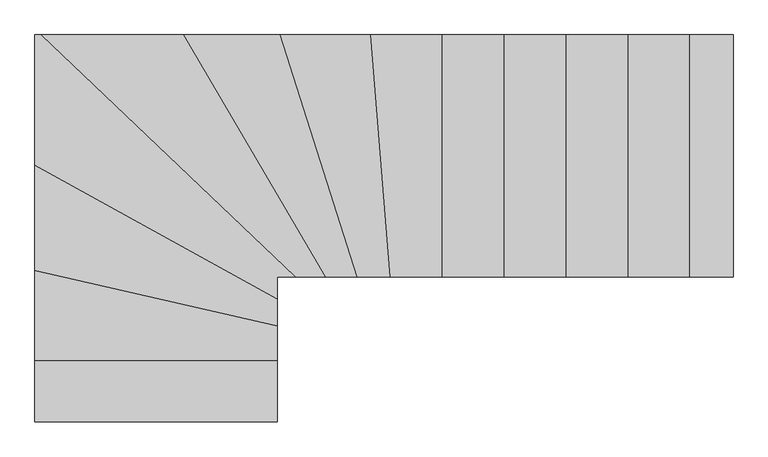
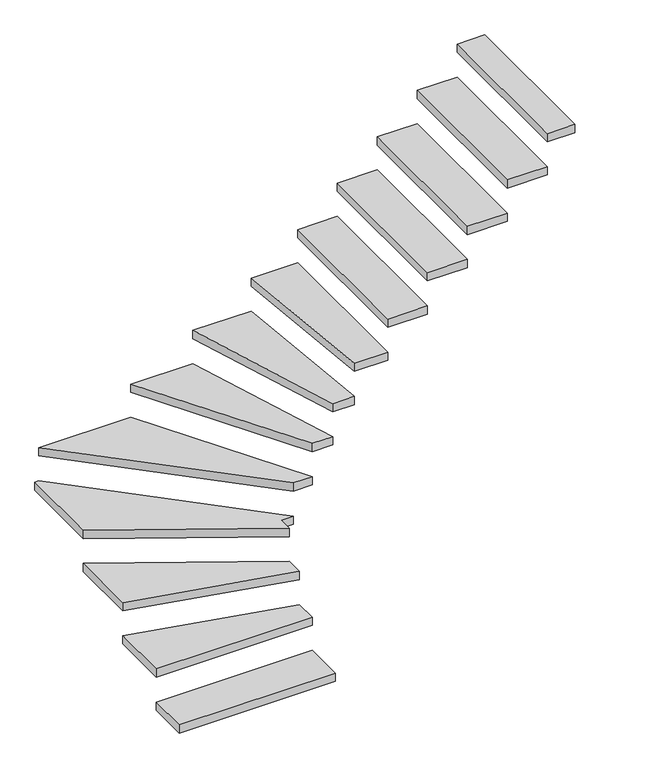
"""IFC4 building model written with IfcOpenShell, lengths in millimetres: stair geometry,   151260 :   151260."""

import ifcopenshell
import ifcopenshell.guid

model = None  # the IFC model being written
_history = None  # IfcOwnerHistory: only IFC2X3 demands one
_inside = {}  # id of a spatial element -> (the spatial element, [elements in it])
_under = {}  # id of a project, library or spatial element -> (it, [spatial elements below it])
_declared = {}  # id of a project -> (the project, [libraries it declares])
_typed = {}  # id of a type object -> (the type object, [elements of that type])
_made_of = {}  # id of a material, layer set ... -> (it, [elements and type objects made of it])


def new_model(schema):
    """Start an empty IFC model of exactly this schema.

    Asked for "IFC4X3", IfcOpenShell would pick the latest addendum, in which some entities
    have other attributes; the version numbers below select the first issue.
    IFC2X3 requires an IfcOwnerHistory on every rooted entity: one is made here for all.
    """
    global model, _history
    if schema == "IFC4X3":
        model = ifcopenshell.file(schema_version=(4, 3, 0, 0))
    else:
        model = ifcopenshell.file(schema=schema)
    _inside.clear()
    _under.clear()
    _declared.clear()
    _typed.clear()
    _made_of.clear()
    _history = None
    if model.schema == "IFC2X3":
        org = make("IfcOrganization", Name="unknown")
        user = make(
            "IfcPersonAndOrganization",
            ThePerson=make("IfcPerson", FamilyName="unknown"),
            TheOrganization=org,
        )
        app = make(
            "IfcApplication",
            ApplicationDeveloper=org,
            Version="unknown",
            ApplicationFullName="unknown",
            ApplicationIdentifier="unknown",
        )
        _history = make(
            "IfcOwnerHistory",
            OwningUser=user,
            OwningApplication=app,
            ChangeAction="ADDED",
            CreationDate=0,
        )
    return model


def make(cls, **values):
    """One entity of the class cls with the attributes given. An attribute that is None is left unset."""
    return model.create_entity(
        cls, **{name: value for name, value in values.items() if value is not None}
    )


def rooted(cls, **values):
    """An entity with a GlobalId (a new one), such as an element, a storey or a relation."""
    return make(cls, GlobalId=ifcopenshell.guid.new(), OwnerHistory=_history, **values)


def si_unit(unit_type, name, prefix=None):
    """IfcSIUnit, for example si_unit("LENGTHUNIT", "METRE", prefix="MILLI")."""
    return make("IfcSIUnit", UnitType=unit_type, Prefix=prefix, Name=name)


def assignment(units):
    """IfcUnitAssignment: the units of a project."""
    return None if units is None else make("IfcUnitAssignment", Units=units)


def point(xyz):
    """IfcCartesianPoint."""
    return None if xyz is None else make("IfcCartesianPoint", Coordinates=xyz)


def direction(xyz):
    """IfcDirection."""
    return None if xyz is None else make("IfcDirection", DirectionRatios=xyz)


def frame(location, z_axis=None, x_axis=None):
    """IfcAxis2Placement3D, a coordinate frame: its origin and axes. An axis left out is left unset."""
    return make(
        "IfcAxis2Placement3D",
        Location=point(location),
        Axis=direction(z_axis),
        RefDirection=direction(x_axis),
    )


def origin():
    """The frame at (0, 0, 0) with its axes left unset."""
    return frame((0.0, 0.0, 0.0))


def place(relative_to, where):
    """IfcLocalPlacement: puts the frame where relative to a parent placement (None: the world)."""
    return make(
        "IfcLocalPlacement", PlacementRelTo=relative_to, RelativePlacement=where
    )


def context(
    kind, dimensions, precision=None, world=None, true_north=None, identifier=None
):
    """IfcGeometricRepresentationContext, for example the 3D "Model" context."""
    return make(
        "IfcGeometricRepresentationContext",
        ContextIdentifier=identifier,
        ContextType=kind,
        CoordinateSpaceDimension=dimensions,
        Precision=precision,
        WorldCoordinateSystem=world,
        TrueNorth=true_north,
    )


def project(units=None, contexts=None):
    """IfcProject with its units and contexts."""
    return rooted(
        "IfcProject",
        Name="project",
        RepresentationContexts=contexts,
        UnitsInContext=assignment(units),
    )


def spatial(cls, under=None, at=None, **own):
    """A site, building, storey or space (cls), placed at a placement, below another one or the project."""
    s = rooted(cls, ObjectPlacement=at, **own)
    if under is not None:
        _under.setdefault(under.id(), (under, []))[1].append(s)
    return s


def polyline(points):
    """IfcPolyline through the points."""
    return make("IfcPolyline", Points=[point(p) for p in points])


def outline(outer, holes=None, kind="AREA"):
    """IfcArbitraryClosedProfileDef: a profile drawn as a closed curve; with holes, ...WithVoids."""
    if holes is None:
        return make("IfcArbitraryClosedProfileDef", ProfileType=kind, OuterCurve=outer)
    return make(
        "IfcArbitraryProfileDefWithVoids",
        ProfileType=kind,
        OuterCurve=outer,
        InnerCurves=holes,
    )


def extrude(swept, where, along, depth):
    """IfcExtrudedAreaSolid: the profile swept, set in the frame where, extruded along a direction by depth."""
    return make(
        "IfcExtrudedAreaSolid",
        SweptArea=swept,
        Position=where,
        ExtrudedDirection=direction(along),
        Depth=depth,
    )


def shape(context_of_items, identifier, shape_type, items):
    """IfcShapeRepresentation: the items that make up one representation, for example the "Body"."""
    return make(
        "IfcShapeRepresentation",
        ContextOfItems=context_of_items,
        RepresentationIdentifier=identifier,
        RepresentationType=shape_type,
        Items=items,
    )


def source(mapping_origin, context_of_items, identifier, shape_type, items):
    """IfcRepresentationMap: a shape defined once, which mapped items show again and again."""
    return make(
        "IfcRepresentationMap",
        MappingOrigin=mapping_origin,
        MappedRepresentation=shape(context_of_items, identifier, shape_type, items),
    )


def transform(
    local_origin,
    x_axis=None,
    y_axis=None,
    z_axis=None,
    scale=None,
    scale2=None,
    scale3=None,
    uniform=True,
):
    """IfcCartesianTransformationOperator3D, or its non-uniform kind. x_axis, y_axis, z_axis: its Axis1, 2, 3."""
    if uniform:
        return make(
            "IfcCartesianTransformationOperator3D",
            Axis1=direction(x_axis),
            Axis2=direction(y_axis),
            LocalOrigin=point(local_origin),
            Scale=scale,
            Axis3=direction(z_axis),
        )
    return make(
        "IfcCartesianTransformationOperator3DnonUniform",
        Axis1=direction(x_axis),
        Axis2=direction(y_axis),
        LocalOrigin=point(local_origin),
        Scale=scale,
        Axis3=direction(z_axis),
        Scale2=scale2,
        Scale3=scale3,
    )


def mapped(mapping_source, mapping_target):
    """IfcMappedItem: shows the shape of a source again, moved by a transform."""
    return make(
        "IfcMappedItem", MappingSource=mapping_source, MappingTarget=mapping_target
    )


def made_of(thing, what):
    """Note that an element or type object is made of a material, layer set ...; save() writes the relation."""
    if what is not None:
        _made_of.setdefault(what.id(), (what, []))[1].append(thing)
    return thing


def element(
    cls,
    number,
    at=None,
    inside=None,
    cuts=None,
    type_object=None,
    material=None,
    context=None,
    identifier="Body",
    shape_type=None,
    held_by="IfcProductDefinitionShape",
    body=None,
    shapes=None,
    **own,
):
    """One element of the class cls, such as IfcWall. Its Tag is "e" and its number.

    at: its placement. inside: the storey or other place that contains it. cuts: it is an
    opening in that element (IfcRelVoidsElement). A single representation is given by context,
    identifier, shape_type and body (its items); several are given by shapes. held_by: the class
    of the entity that holds the representations. save() writes the other relations.
    """
    e = rooted(cls, Tag="e%d" % number, ObjectPlacement=at, **own)
    if body is not None:
        shapes = [shape(context, identifier, shape_type, body)]
    if shapes is not None:
        e.Representation = make(held_by, Representations=shapes)
    if inside is not None:
        _inside.setdefault(inside.id(), (inside, []))[1].append(e)
    if cuts is not None:
        rooted(
            "IfcRelVoidsElement", RelatingBuildingElement=cuts, RelatedOpeningElement=e
        )
    if type_object is not None:
        _typed.setdefault(type_object.id(), (type_object, []))[1].append(e)
    return made_of(e, material)


def aggregate(whole, parts):
    """IfcRelAggregates: a whole, such as a stair, and the parts it consists of."""
    return rooted("IfcRelAggregates", RelatingObject=whole, RelatedObjects=parts)


def save(model, path):
    """Write the relations noted so far, then the file.

    IfcRelAggregates (storeys below a building ...), IfcRelContainedInSpatialStructure (elements
    in a storey), IfcRelDefinesByType, IfcRelAssociatesMaterial and IfcRelDeclares: one each for
    every whole, place, type object, material and project.
    """
    for whole, parts in _under.values():
        aggregate(whole, parts)
    for where, things in _inside.values():
        rooted(
            "IfcRelContainedInSpatialStructure",
            RelatedElements=things,
            RelatingStructure=where,
        )
    for kind, things in _typed.values():
        rooted("IfcRelDefinesByType", RelatedObjects=things, RelatingType=kind)
    for what, things in _made_of.values():
        rooted("IfcRelAssociatesMaterial", RelatedObjects=things, RelatingMaterial=what)
    for by, libraries in _declared.values():
        rooted("IfcRelDeclares", RelatingContext=by, RelatedDefinitions=libraries)
    model.write(path)


def stair_4856ba97(model_context):
    return source(origin(), model_context, "Body", "SweptSolid", [
        extrude(outline(polyline([(159177.7593015, 39074.7962965), (160077.7593015, 39074.7962965), (160077.7593015, 38844.7962965), (159177.7593015, 38844.7962965), (159177.7593015, 39074.7962965)])), frame((0.0, 0.0, 3482.1428571), z_axis=(0.0, 0.0, 1.0), x_axis=(1.0, 0.0, 0.0)), (0.0, 0.0, 1.0), 50.0),
        extrude(outline(polyline([(159177.7593015, 39407.7634868), (160077.7593015, 39201.8291061), (160077.7593015, 39074.7962965), (159177.7593015, 39074.7962965), (159177.7593015, 39407.7634868)])), frame((0.0, 0.0, 3684.2857143), z_axis=(0.0, 0.0, 1.0), x_axis=(1.0, 0.0, 0.0)), (0.0, 0.0, 1.0), 50.0),
        extrude(outline(polyline([(159177.7593015, 39801.0914939), (160077.7593015, 39301.7193734), (160077.7593015, 39201.8291061), (159177.7593015, 39407.7634868), (159177.7593015, 39801.0914939)])), frame((0.0, 0.0, 3886.4285714), z_axis=(0.0, 0.0, 1.0), x_axis=(1.0, 0.0, 0.0)), (0.0, 0.0, 1.0), 50.0),
        extrude(outline(polyline([(159177.7593015, 40284.7962965), (159200.4297176, 40284.7962965), (160147.7593015, 39384.7962965), (160077.7593015, 39384.7962965), (160077.7593015, 39301.7193734), (159177.7593015, 39801.0914939), (159177.7593015, 40284.7962965)])), frame((0.0, 0.0, 4088.5714286), z_axis=(0.0, 0.0, 1.0), x_axis=(1.0, 0.0, 0.0)), (0.0, 0.0, 1.0), 50.0),
        extrude(outline(polyline([(159730.1980238, 40284.7962965), (160258.7713888, 39384.7962965), (160147.7593015, 39384.7962965), (159200.4297176, 40284.7962965), (159730.1980238, 40284.7962965)])), frame((0.0, 0.0, 4290.7142857), z_axis=(0.0, 0.0, 1.0), x_axis=(1.0, 0.0, 0.0)), (0.0, 0.0, 1.0), 50.0),
        extrude(outline(polyline([(160089.4284981, 40284.7962965), (160375.293778, 39384.7962965), (160258.7713888, 39384.7962965), (159730.1980238, 40284.7962965), (160089.4284981, 40284.7962965)])), frame((0.0, 0.0, 4492.8571429), z_axis=(0.0, 0.0, 1.0), x_axis=(1.0, 0.0, 0.0)), (0.0, 0.0, 1.0), 50.0),
        extrude(outline(polyline([(160425.6183342, 40284.7962965), (160499.1039419, 39384.7962965), (160375.293778, 39384.7962965), (160089.4284981, 40284.7962965), (160425.6183342, 40284.7962965)])), frame((0.0, 0.0, 4695.0), z_axis=(0.0, 0.0, 1.0), x_axis=(1.0, 0.0, 0.0)), (0.0, 0.0, 1.0), 50.0),
        extrude(outline(polyline([(160692.3611381, 40284.7962965), (160692.3611381, 39384.7962965), (160499.1039419, 39384.7962965), (160425.6183342, 40284.7962965), (160692.3611381, 40284.7962965)])), frame((0.0, 0.0, 4897.1428571), z_axis=(0.0, 0.0, 1.0), x_axis=(1.0, 0.0, 0.0)), (0.0, 0.0, 1.0), 50.0),
        extrude(outline(polyline([(160922.3611381, 40284.7962965), (160922.3611381, 39384.7962965), (160692.3611381, 39384.7962965), (160692.3611381, 40284.7962965), (160922.3611381, 40284.7962965)])), frame((0.0, 0.0, 5099.2857143), z_axis=(0.0, 0.0, 1.0), x_axis=(1.0, 0.0, 0.0)), (0.0, 0.0, 1.0), 50.0),
        extrude(outline(polyline([(161152.3611381, 40284.7962965), (161152.3611381, 39384.7962965), (160922.3611381, 39384.7962965), (160922.3611381, 40284.7962965), (161152.3611381, 40284.7962965)])), frame((0.0, 0.0, 5301.4285714), z_axis=(0.0, 0.0, 1.0), x_axis=(1.0, 0.0, 0.0)), (0.0, 0.0, 1.0), 50.0),
        extrude(outline(polyline([(161382.3611381, 40284.7962965), (161382.3611381, 39384.7962965), (161152.3611381, 39384.7962965), (161152.3611381, 40284.7962965), (161382.3611381, 40284.7962965)])), frame((0.0, 0.0, 5503.5714286), z_axis=(0.0, 0.0, 1.0), x_axis=(1.0, 0.0, 0.0)), (0.0, 0.0, 1.0), 50.0),
        extrude(outline(polyline([(161612.3611381, 40284.7962965), (161612.3611381, 39384.7962965), (161382.3611381, 39384.7962965), (161382.3611381, 40284.7962965), (161612.3611381, 40284.7962965)])), frame((0.0, 0.0, 5705.7142857), z_axis=(0.0, 0.0, 1.0), x_axis=(1.0, 0.0, 0.0)), (0.0, 0.0, 1.0), 50.0),
        extrude(outline(polyline([(161772.7593015, 40284.7962965), (161772.7593015, 39384.7962965), (161612.3611381, 39384.7962965), (161612.3611381, 40284.7962965), (161772.7593015, 40284.7962965)])), frame((0.0, 0.0, 5907.8571429), z_axis=(0.0, 0.0, 1.0), x_axis=(1.0, 0.0, 0.0)), (0.0, 0.0, 1.0), 50.0),
    ])


if __name__ == "__main__":
    model = new_model("IFC4")
    model_context = context("Model", 3, world=origin())
    ifc_project = project(units=[si_unit("LENGTHUNIT", "METRE", prefix="MILLI")], contexts=[model_context])
    site = spatial("IfcSite", under=ifc_project)
    building = spatial("IfcBuilding", under=site)
    placement = place(None, origin())
    stair_shape = stair_4856ba97(model_context)
    element("IfcStair", 1, ObjectType="  151260 :   151260", at=placement, inside=building, context=model_context, shape_type="MappedRepresentation", body=[
        mapped(stair_shape, transform((0.0, 0.0, 0.0), x_axis=(1.0, 0.0, 0.0), y_axis=(0.0, 1.0, 0.0), z_axis=(0.0, 0.0, 1.0))),
    ])
    save(model, "model.ifc")

# Revit data of these elements
# Type "  151260 :   151260"
#   Abrechnungsart = "St"
#   Allright_Bauteil_ID = "0131Tre0659044533"
#   Material = "Stahlbeton"
#   Objektname = "Treppe"
#   NameOverride = " "
#   ThermalTransmittance = 0.0000 BTU/(h·ft²·°F)
#   NosingLength = 0.000 m
#   NumberOfRiser = 14
#   NumberOfTreads = 13
#   RiserHeight = 2.021 m
#   TreadLength = 2.300 m
#   IsExternal = no
#   FireExit = no
#   HandicapAccessible = no
#   HasNonSkidSurface = no
# Element 1 (IfcStair, "  151260 :   151260")
#   Materials on its faces: "weiss"
# Materials
#   "weiss": class "Unassigned", colour RGB 255 255 255, transparency 0
